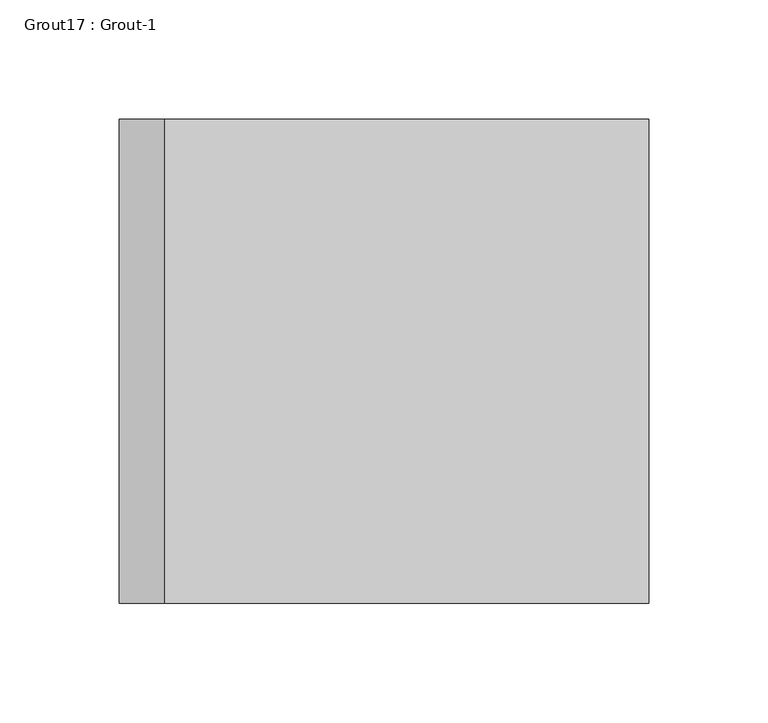
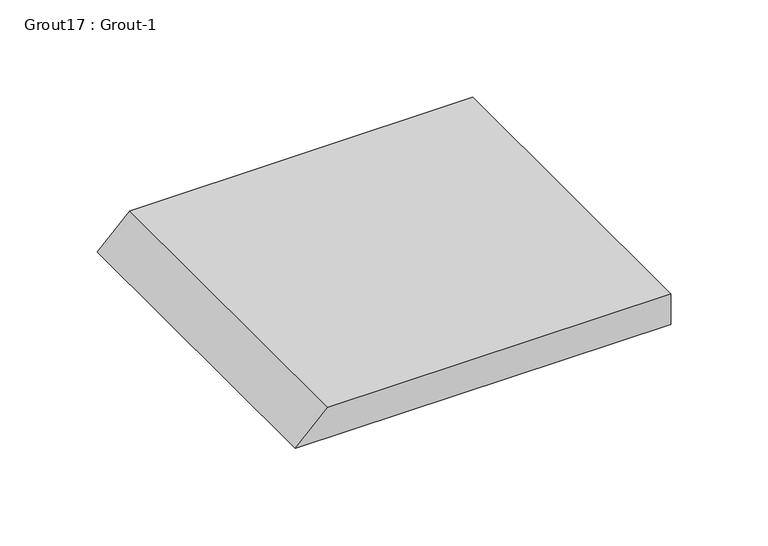
"""IFC4 building model written with IfcOpenShell, lengths in millimetres: proxy geometry, Grout17 : Grout-1."""

from ifc_helpers import new_model, si_unit, frame, origin, place, context, project, spatial, polyline, outline, extrude, source, transform, mapped, element, save


def grout17_grout_1_0f871906(model_context):
    return source(origin(), model_context, "Body", "SweptSolid", [
        extrude(outline(polyline([(19.05, 590115.4434739), (0.0, 590096.3934739), (0.0, 590318.6434739), (19.05, 590318.6434739), (19.05, 590115.4434739)])), frame((0.0, -535306.3413841, 0.0), z_axis=(0.0, 1.0, 0.0), x_axis=(0.0, 0.0, 1.0)), (0.0, 0.0, 1.0), 203.2),
    ])


if __name__ == "__main__":
    model = new_model("IFC4")
    model_context = context("Model", 3, world=origin())
    ifc_project = project(units=[si_unit("LENGTHUNIT", "METRE", prefix="MILLI")], contexts=[model_context])
    site = spatial("IfcSite", under=ifc_project)
    building = spatial("IfcBuilding", under=site)
    placement = place(None, origin())
    grout17_grout_1_shape = grout17_grout_1_0f871906(model_context)
    element("IfcBuildingElementProxy", 1, Name="Grout17 : Grout-1", ObjectType="Grout17 : Grout-1", at=placement, inside=building, context=model_context, shape_type="MappedRepresentation", body=[
        mapped(grout17_grout_1_shape, transform((0.0, 0.0, 0.0), x_axis=(1.0, 0.0, 0.0), y_axis=(0.0, 1.0, 0.0), z_axis=(0.0, 0.0, 1.0))),
    ])
    save(model, "model.ifc")

# Revit data of these elements
# Element 1 (IfcBuildingElementProxy, "Grout17 : Grout-1")
#   Materials on its faces: "3/4\" NON SHRINK GROUT"
# Materials
#   "3/4\" NON SHRINK GROUT": class "Generic", colour RGB 145 145 143, transparency 0, Cost = 0
